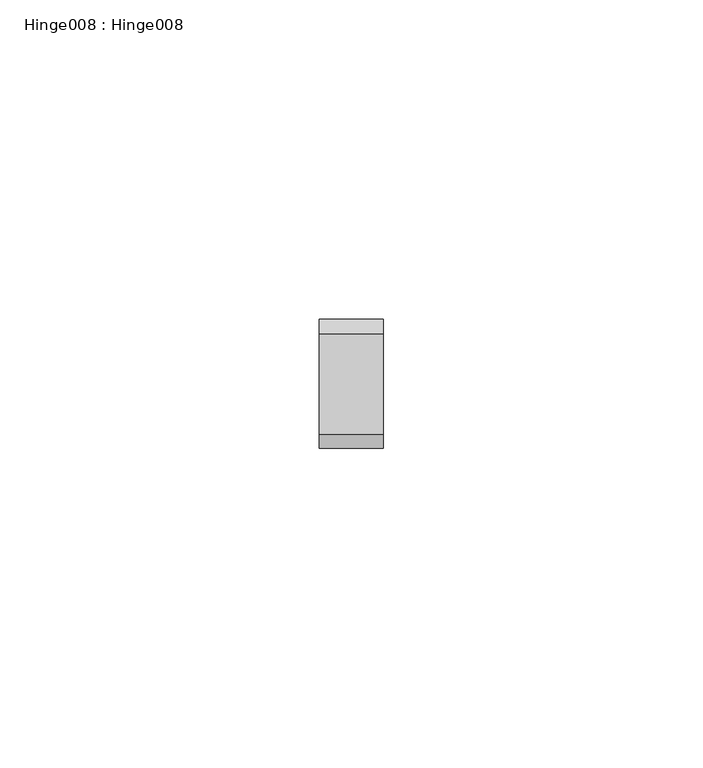
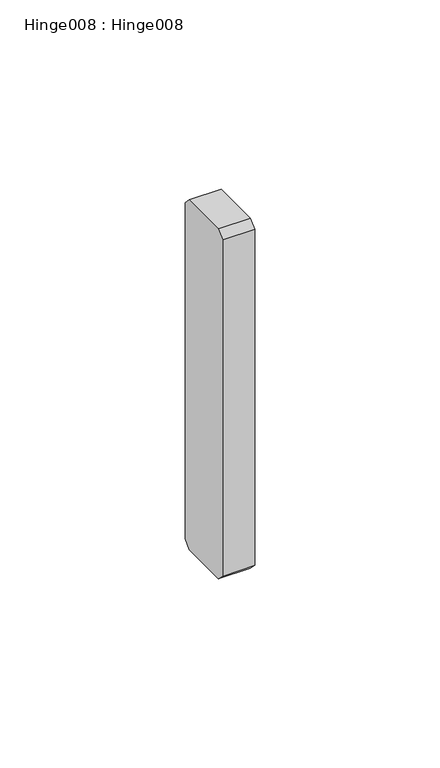
"""IFC4 building model written with IfcOpenShell, lengths in millimetres: proxy geometry, Hinge008 : Hinge008."""

from ifc_helpers import new_model, si_unit, frame, origin, place, context, project, spatial, polyline, outline, extrude, source, transform, mapped, element, save


def hinge008_hinge008_00bb6158(model_context):
    return source(origin(), model_context, "Body", "SweptSolid", [
        extrude(outline(polyline([(9646.679882, 37769.0012561), (9630.9579547, 37769.0012561), (9628.7124545, 37771.2467563), (9628.7124545, 37882.1452438), (9630.9579547, 37884.3907439), (9646.679882, 37884.3907439), (9648.924946, 37882.1456799), (9648.924946, 37771.2463201), (9646.679882, 37769.0012561)])), frame((-7242.2219278, 0.0, 0.0), z_axis=(1.0, 0.0, 0.0), x_axis=(0.0, 1.0, 0.0)), (0.0, 0.0, 1.0), 10.0),
    ])


if __name__ == "__main__":
    model = new_model("IFC4")
    model_context = context("Model", 3, world=origin())
    ifc_project = project(units=[si_unit("LENGTHUNIT", "METRE", prefix="MILLI")], contexts=[model_context])
    site = spatial("IfcSite", under=ifc_project)
    building = spatial("IfcBuilding", under=site)
    placement = place(None, origin())
    hinge008_hinge008_shape = hinge008_hinge008_00bb6158(model_context)
    element("IfcBuildingElementProxy", 1, Name="Hinge008 : Hinge008", ObjectType="Hinge008 : Hinge008", at=placement, inside=building, context=model_context, shape_type="MappedRepresentation", body=[
        mapped(hinge008_hinge008_shape, transform((0.0, 0.0, 0.0), x_axis=(1.0, 0.0, 0.0), y_axis=(0.0, 1.0, 0.0), z_axis=(0.0, 0.0, 1.0))),
    ])
    save(model, "model.ifc")

# Revit data of these elements
# Type "Hinge008 : Hinge008"
#   NameOverride = "Hinge008"
# Element 1 (IfcBuildingElementProxy, "Hinge008 : Hinge008")
#   Materials on its faces: "HEAVY DUTY STAINLESS STEEL HINGE (90 DEGREE ROTATION)"
# Materials
#   "HEAVY DUTY STAINLESS STEEL HINGE (90 DEGREE ROTATION)": class "Unassigned", colour RGB 128 128 128, transparency 0
